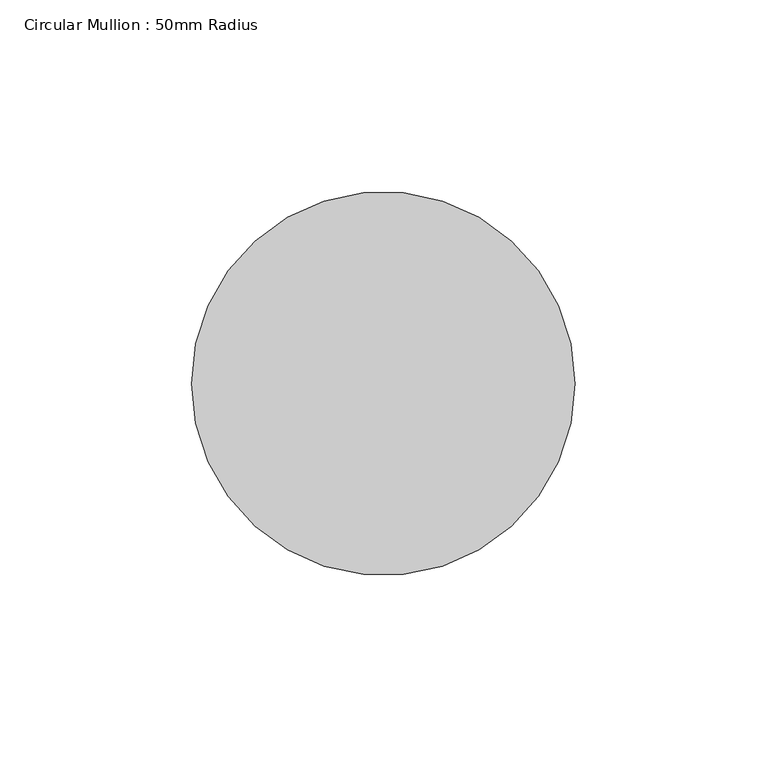
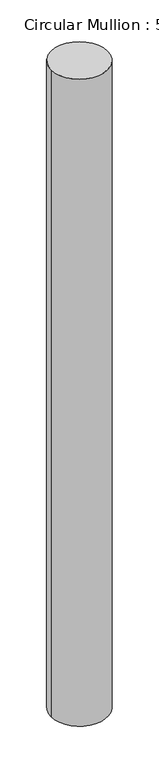
"""IFC4 building model written with IfcOpenShell, lengths in millimetres: member geometry, Circular Mullion : 50mm Radius."""

from ifc_helpers import new_model, si_unit, point, frame, origin, origin_2d, place, context, project, spatial, circle_curve, trimmed, segment, composite_curve, outline, extrude, source, transform, mapped, element, save


def circular_mullion_50mm_radius_4ba2d17e(model_context):
    return source(origin(), model_context, "Body", "SweptSolid", [
        extrude(outline(composite_curve([segment(trimmed(circle_curve(origin_2d(), 50.0), [point((50.0, 0.0))], [point((-50.0, 0.0))], False, "CARTESIAN"), True, "CONTINUOUS"), segment(trimmed(circle_curve(origin_2d(), 50.0), [point((-50.0, 0.0))], [point((50.0, 0.0))], False, "CARTESIAN"), True, "CONTINUOUS")], self_intersect=False)), frame((0.0, 0.0, -1208.7794767), z_axis=(0.0, 0.0, 1.0), x_axis=(1.0, 0.0, 0.0)), (0.0, 0.0, 1.0), 1208.7794767),
    ])


if __name__ == "__main__":
    model = new_model("IFC4")
    model_context = context("Model", 3, world=origin())
    ifc_project = project(units=[si_unit("LENGTHUNIT", "METRE", prefix="MILLI")], contexts=[model_context])
    site = spatial("IfcSite", under=ifc_project)
    building = spatial("IfcBuilding", under=site)
    placement = place(None, origin())
    circular_mullion_50mm_radius_shape = circular_mullion_50mm_radius_4ba2d17e(model_context)
    element("IfcMember", 1, ObjectType="Circular Mullion : 50mm Radius", at=placement, inside=building, context=model_context, shape_type="MappedRepresentation", body=[
        mapped(circular_mullion_50mm_radius_shape, transform((0.0, 0.0, 0.0), x_axis=(1.0, 0.0, 0.0), y_axis=(0.0, 1.0, 0.0), z_axis=(0.0, 0.0, 1.0))),
    ])
    save(model, "model.ifc")

# Revit data of these elements
# Type "Circular Mullion : 50mm Radius"
#   built-in parameter 1007350 = 0.164042 (stored number, unit not read)
# Element 1 (IfcMember, "Circular Mullion : 50mm Radius")
#   Materials on its faces: "Aluminium"
# Materials
#   "Aluminium": class "Metal", colour RGB 247 247 247, transparency 0, Description = "Aluminium 6061", Cost = 0
